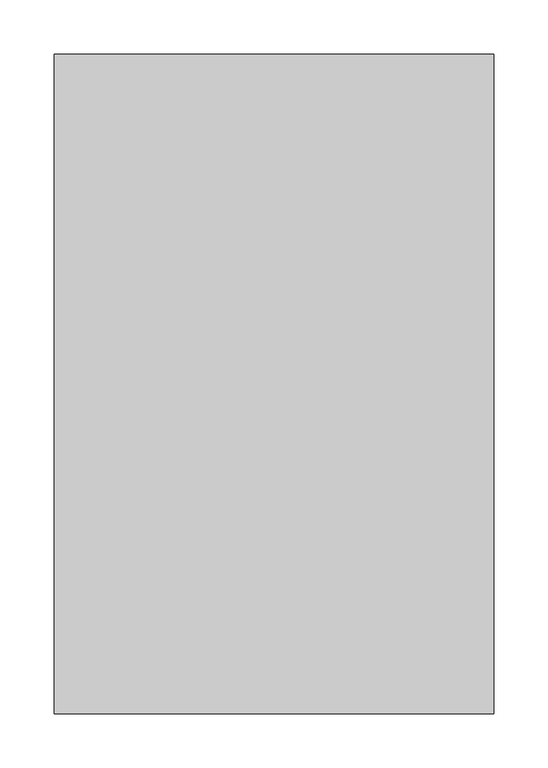
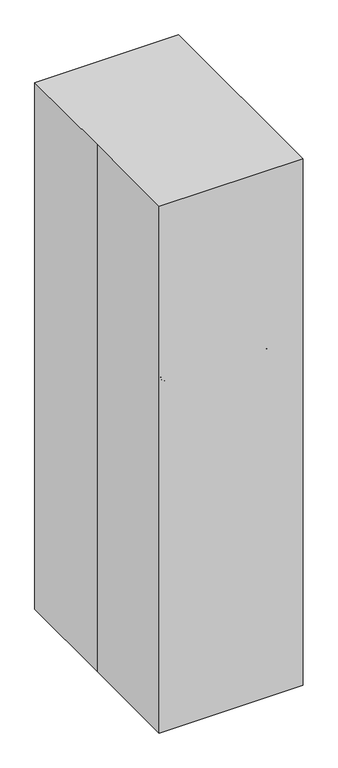
"""IFC4 building model written with IfcOpenShell, lengths in millimetres: proxy geometry, M8810 - Stand, Mayo : M8810 - Stand, Mayo."""

import ifcopenshell
import ifcopenshell.guid

model = None  # the IFC model being written
_history = None  # IfcOwnerHistory: only IFC2X3 demands one
_inside = {}  # id of a spatial element -> (the spatial element, [elements in it])
_under = {}  # id of a project, library or spatial element -> (it, [spatial elements below it])
_declared = {}  # id of a project -> (the project, [libraries it declares])
_typed = {}  # id of a type object -> (the type object, [elements of that type])
_made_of = {}  # id of a material, layer set ... -> (it, [elements and type objects made of it])


def new_model(schema):
    """Start an empty IFC model of exactly this schema.

    Asked for "IFC4X3", IfcOpenShell would pick the latest addendum, in which some entities
    have other attributes; the version numbers below select the first issue.
    IFC2X3 requires an IfcOwnerHistory on every rooted entity: one is made here for all.
    """
    global model, _history
    if schema == "IFC4X3":
        model = ifcopenshell.file(schema_version=(4, 3, 0, 0))
    else:
        model = ifcopenshell.file(schema=schema)
    _inside.clear()
    _under.clear()
    _declared.clear()
    _typed.clear()
    _made_of.clear()
    _history = None
    if model.schema == "IFC2X3":
        org = make("IfcOrganization", Name="unknown")
        user = make(
            "IfcPersonAndOrganization",
            ThePerson=make("IfcPerson", FamilyName="unknown"),
            TheOrganization=org,
        )
        app = make(
            "IfcApplication",
            ApplicationDeveloper=org,
            Version="unknown",
            ApplicationFullName="unknown",
            ApplicationIdentifier="unknown",
        )
        _history = make(
            "IfcOwnerHistory",
            OwningUser=user,
            OwningApplication=app,
            ChangeAction="ADDED",
            CreationDate=0,
        )
    return model


def make(cls, **values):
    """One entity of the class cls with the attributes given. An attribute that is None is left unset."""
    return model.create_entity(
        cls, **{name: value for name, value in values.items() if value is not None}
    )


def rooted(cls, **values):
    """An entity with a GlobalId (a new one), such as an element, a storey or a relation."""
    return make(cls, GlobalId=ifcopenshell.guid.new(), OwnerHistory=_history, **values)


def si_unit(unit_type, name, prefix=None):
    """IfcSIUnit, for example si_unit("LENGTHUNIT", "METRE", prefix="MILLI")."""
    return make("IfcSIUnit", UnitType=unit_type, Prefix=prefix, Name=name)


def assignment(units):
    """IfcUnitAssignment: the units of a project."""
    return None if units is None else make("IfcUnitAssignment", Units=units)


def point(xyz):
    """IfcCartesianPoint."""
    return None if xyz is None else make("IfcCartesianPoint", Coordinates=xyz)


def direction(xyz):
    """IfcDirection."""
    return None if xyz is None else make("IfcDirection", DirectionRatios=xyz)


def frame(location, z_axis=None, x_axis=None):
    """IfcAxis2Placement3D, a coordinate frame: its origin and axes. An axis left out is left unset."""
    return make(
        "IfcAxis2Placement3D",
        Location=point(location),
        Axis=direction(z_axis),
        RefDirection=direction(x_axis),
    )


def origin():
    """The frame at (0, 0, 0) with its axes left unset."""
    return frame((0.0, 0.0, 0.0))


def origin_with_axes():
    """The frame at (0, 0, 0) with the z axis (0, 0, 1) and the x axis (1, 0, 0) written out."""
    return frame((0.0, 0.0, 0.0), z_axis=(0.0, 0.0, 1.0), x_axis=(1.0, 0.0, 0.0))


def place(relative_to, where):
    """IfcLocalPlacement: puts the frame where relative to a parent placement (None: the world)."""
    return make(
        "IfcLocalPlacement", PlacementRelTo=relative_to, RelativePlacement=where
    )


def context(
    kind, dimensions, precision=None, world=None, true_north=None, identifier=None
):
    """IfcGeometricRepresentationContext, for example the 3D "Model" context."""
    return make(
        "IfcGeometricRepresentationContext",
        ContextIdentifier=identifier,
        ContextType=kind,
        CoordinateSpaceDimension=dimensions,
        Precision=precision,
        WorldCoordinateSystem=world,
        TrueNorth=true_north,
    )


def project(units=None, contexts=None):
    """IfcProject with its units and contexts."""
    return rooted(
        "IfcProject",
        Name="project",
        RepresentationContexts=contexts,
        UnitsInContext=assignment(units),
    )


def spatial(cls, under=None, at=None, **own):
    """A site, building, storey or space (cls), placed at a placement, below another one or the project."""
    s = rooted(cls, ObjectPlacement=at, **own)
    if under is not None:
        _under.setdefault(under.id(), (under, []))[1].append(s)
    return s


def polyline(points):
    """IfcPolyline through the points."""
    return make("IfcPolyline", Points=[point(p) for p in points])


def circle_curve(where, radius):
    """IfcCircle in the frame where."""
    return make("IfcCircle", Position=where, Radius=radius)


def ellipse_curve(where, semi_axis1, semi_axis2):
    """IfcEllipse in the frame where."""
    return make(
        "IfcEllipse", Position=where, SemiAxis1=semi_axis1, SemiAxis2=semi_axis2
    )


def trimmed(basis, trim1, trim2, sense, master):
    """IfcTrimmedCurve: the piece of a basis curve between two trims."""
    return make(
        "IfcTrimmedCurve",
        BasisCurve=basis,
        Trim1=trim1,
        Trim2=trim2,
        SenseAgreement=sense,
        MasterRepresentation=master,
    )


def outline(outer, holes=None, kind="AREA"):
    """IfcArbitraryClosedProfileDef: a profile drawn as a closed curve; with holes, ...WithVoids."""
    if holes is None:
        return make("IfcArbitraryClosedProfileDef", ProfileType=kind, OuterCurve=outer)
    return make(
        "IfcArbitraryProfileDefWithVoids",
        ProfileType=kind,
        OuterCurve=outer,
        InnerCurves=holes,
    )


def extrude(swept, where, along, depth):
    """IfcExtrudedAreaSolid: the profile swept, set in the frame where, extruded along a direction by depth."""
    return make(
        "IfcExtrudedAreaSolid",
        SweptArea=swept,
        Position=where,
        ExtrudedDirection=direction(along),
        Depth=depth,
    )


def shape(context_of_items, identifier, shape_type, items):
    """IfcShapeRepresentation: the items that make up one representation, for example the "Body"."""
    return make(
        "IfcShapeRepresentation",
        ContextOfItems=context_of_items,
        RepresentationIdentifier=identifier,
        RepresentationType=shape_type,
        Items=items,
    )


def source(mapping_origin, context_of_items, identifier, shape_type, items):
    """IfcRepresentationMap: a shape defined once, which mapped items show again and again."""
    return make(
        "IfcRepresentationMap",
        MappingOrigin=mapping_origin,
        MappedRepresentation=shape(context_of_items, identifier, shape_type, items),
    )


def transform(
    local_origin,
    x_axis=None,
    y_axis=None,
    z_axis=None,
    scale=None,
    scale2=None,
    scale3=None,
    uniform=True,
):
    """IfcCartesianTransformationOperator3D, or its non-uniform kind. x_axis, y_axis, z_axis: its Axis1, 2, 3."""
    if uniform:
        return make(
            "IfcCartesianTransformationOperator3D",
            Axis1=direction(x_axis),
            Axis2=direction(y_axis),
            LocalOrigin=point(local_origin),
            Scale=scale,
            Axis3=direction(z_axis),
        )
    return make(
        "IfcCartesianTransformationOperator3DnonUniform",
        Axis1=direction(x_axis),
        Axis2=direction(y_axis),
        LocalOrigin=point(local_origin),
        Scale=scale,
        Axis3=direction(z_axis),
        Scale2=scale2,
        Scale3=scale3,
    )


def mapped(mapping_source, mapping_target):
    """IfcMappedItem: shows the shape of a source again, moved by a transform."""
    return make(
        "IfcMappedItem", MappingSource=mapping_source, MappingTarget=mapping_target
    )


def made_of(thing, what):
    """Note that an element or type object is made of a material, layer set ...; save() writes the relation."""
    if what is not None:
        _made_of.setdefault(what.id(), (what, []))[1].append(thing)
    return thing


def element(
    cls,
    number,
    at=None,
    inside=None,
    cuts=None,
    type_object=None,
    material=None,
    context=None,
    identifier="Body",
    shape_type=None,
    held_by="IfcProductDefinitionShape",
    body=None,
    shapes=None,
    **own,
):
    """One element of the class cls, such as IfcWall. Its Tag is "e" and its number.

    at: its placement. inside: the storey or other place that contains it. cuts: it is an
    opening in that element (IfcRelVoidsElement). A single representation is given by context,
    identifier, shape_type and body (its items); several are given by shapes. held_by: the class
    of the entity that holds the representations. save() writes the other relations.
    """
    e = rooted(cls, Tag="e%d" % number, ObjectPlacement=at, **own)
    if body is not None:
        shapes = [shape(context, identifier, shape_type, body)]
    if shapes is not None:
        e.Representation = make(held_by, Representations=shapes)
    if inside is not None:
        _inside.setdefault(inside.id(), (inside, []))[1].append(e)
    if cuts is not None:
        rooted(
            "IfcRelVoidsElement", RelatingBuildingElement=cuts, RelatedOpeningElement=e
        )
    if type_object is not None:
        _typed.setdefault(type_object.id(), (type_object, []))[1].append(e)
    return made_of(e, material)


def aggregate(whole, parts):
    """IfcRelAggregates: a whole, such as a stair, and the parts it consists of."""
    return rooted("IfcRelAggregates", RelatingObject=whole, RelatedObjects=parts)


def save(model, path):
    """Write the relations noted so far, then the file.

    IfcRelAggregates (storeys below a building ...), IfcRelContainedInSpatialStructure (elements
    in a storey), IfcRelDefinesByType, IfcRelAssociatesMaterial and IfcRelDeclares: one each for
    every whole, place, type object, material and project.
    """
    for whole, parts in _under.values():
        aggregate(whole, parts)
    for where, things in _inside.values():
        rooted(
            "IfcRelContainedInSpatialStructure",
            RelatedElements=things,
            RelatingStructure=where,
        )
    for kind, things in _typed.values():
        rooted("IfcRelDefinesByType", RelatedObjects=things, RelatingType=kind)
    for what, things in _made_of.values():
        rooted("IfcRelAssociatesMaterial", RelatedObjects=things, RelatingMaterial=what)
    for by, libraries in _declared.values():
        rooted("IfcRelDeclares", RelatingContext=by, RelatedDefinitions=libraries)
    model.write(path)


def plane_surface(at):
    """IfcPlane: the flat surface through the origin of the frame at, square to its z axis."""
    return make("IfcPlane", Position=at)


def cylinder_surface(at, radius):
    """IfcCylindricalSurface: all points at the distance radius from the z axis of the frame at."""
    return make("IfcCylindricalSurface", Position=at, Radius=radius)


def revolved_surface(curve, axis_point, axis_direction):
    """IfcSurfaceOfRevolution: the curve turned about the line through axis_point along axis_direction."""
    return make(
        "IfcSurfaceOfRevolution",
        SweptCurve=make("IfcArbitraryOpenProfileDef", ProfileType="CURVE", Curve=curve),
        AxisPosition=make("IfcAxis1Placement", Location=point(axis_point), Axis=direction(axis_direction)),
    )


def advanced_brep(points, edges, surfaces, faces):
    """IfcAdvancedBrep: a solid bounded by faces that lie on surfaces and meet in shared edges.

    An edge is (start, end): straight between two places in points (the first is 0);
    or (start, end, curve); or (start, end, curve, False) where it runs against its curve.
    A face is (place in surfaces, loops), or (place, loops, False) where it looks against
    its surface's normal. A loop lists edges by number (the first is 1), with a minus sign
    where the edge is run from its end to its start. The first loop is the outer one.
    """
    corners = [point(p) for p in points]
    vertices = [make("IfcVertexPoint", VertexGeometry=c) for c in corners]
    made = []
    for start, end, *more in edges:
        made.append(
            make(
                "IfcEdgeCurve",
                EdgeStart=vertices[start],
                EdgeEnd=vertices[end],
                EdgeGeometry=more[0] if more else make("IfcPolyline", Points=[corners[start], corners[end]]),
                SameSense=more[1] if len(more) > 1 else True,
            )
        )
    hull = []
    for where, loops, *sense in faces:
        bounds = []
        for j, loop in enumerate(loops):
            ring = [make("IfcOrientedEdge", EdgeElement=made[abs(k) - 1], Orientation=k > 0) for k in loop]
            bounds.append(
                make(
                    "IfcFaceOuterBound" if j == 0 else "IfcFaceBound",
                    Bound=make("IfcEdgeLoop", EdgeList=ring),
                    Orientation=True,
                )
            )
        hull.append(make("IfcAdvancedFace", Bounds=bounds, FaceSurface=surfaces[where], SameSense=sense[0] if sense else True))
    return make("IfcAdvancedBrep", Outer=make("IfcClosedShell", CfsFaces=hull))


def specialty_equipment_9fd3930d(model_context):
    return source(origin(), model_context, "Body", "SolidModel", [
        advanced_brep(
        [(-123.5140783, 201.8552552, 999.8159151), (-136.2140783, 189.1552552, 999.8159151), (-136.2140783, 189.1552552, 996.6409151), (-123.5140783, 201.8552552, 996.6409151), (-123.5140783, 224.0802552, 1002.9909151), (-158.4390783, 189.1552552, 1002.9909151), (-155.2640783, 189.1552552, 999.8159151), (-123.5140783, 220.9052552, 999.8159151), (-123.5140783, 224.0802552, 1015.2574617), (-158.4390783, 189.1552552, 1015.2574617), (-123.5140783, 226.4102935, 1017.5875), (-160.7691166, 189.1552552, 1017.5875), (-123.5140783, 233.6052552, 1015.5808485), (-167.9640783, 189.1552552, 1015.5808485), (-165.9574268, 189.1552552, 1017.5875), (-123.5140783, 231.5986038, 1017.5875), (-123.5140783, 233.6052552, 1011.9917262), (-167.9640783, 189.1552552, 1011.9917262), (-123.5140783, 232.8510291, 1011.2375), (-167.2098521, 189.1552552, 1011.2375), (-123.5140783, 232.0177552, 1016.0), (-166.3765783, 189.1552552, 1016.0), (-166.3765783, 189.1552552, 1011.2375), (-123.5140783, 232.0177552, 1011.2375), (-123.5140783, 227.2552552, 1002.9909151), (-161.6140783, 189.1552552, 1002.9909151), (-161.6140783, 189.1552552, 1016.0), (-123.5140783, 227.2552552, 1016.0), (-123.5140783, 220.9052552, 996.6409151), (-155.2640783, 189.1552552, 996.6409151), (124.1359217, 201.8552552, 996.6409151), (124.1359217, 201.8552552, 999.8159151), (124.1359217, 220.9052552, 999.8159151), (124.1359217, 224.0802552, 1002.9909151), (124.1359217, 224.0802552, 1015.2574617), (124.1359217, 226.4102935, 1017.5875), (124.1359217, 231.5986038, 1017.5875), (124.1359217, 233.6052552, 1015.5808485), (124.1359217, 233.6052552, 1011.9917262), (124.1359217, 232.8510291, 1011.2375), (124.1359217, 232.0177552, 1011.2375), (124.1359217, 232.0177552, 1016.0), (124.1359217, 227.2552552, 1016.0), (124.1359217, 227.2552552, 1002.9909151), (124.1359217, 220.9052552, 996.6409151), (136.8359217, 189.1552552, 999.8159151), (136.8359217, 189.1552552, 996.6409151), (159.0609217, 189.1552552, 1002.9909151), (155.8859217, 189.1552552, 999.8159151), (159.0609217, 189.1552552, 1015.2574617), (161.39096, 189.1552552, 1017.5875), (168.5859217, 189.1552552, 1015.5808485), (166.5792702, 189.1552552, 1017.5875), (168.5859217, 189.1552552, 1011.9917262), (167.8316955, 189.1552552, 1011.2375), (166.9984217, 189.1552552, 1016.0), (166.9984217, 189.1552552, 1011.2375), (162.2359217, 189.1552552, 1002.9909151), (162.2359217, 189.1552552, 1016.0), (155.8859217, 189.1552552, 996.6409151), (136.8359217, -223.5947448, 996.6409151), (136.8359217, -223.5947448, 999.8159151), (155.8859217, -223.5947448, 999.8159151), (159.0609217, -223.5947448, 1002.9909151), (159.0609217, -223.5947448, 1015.2574617), (161.39096, -223.5947448, 1017.5875), (166.5792702, -223.5947448, 1017.5875), (168.5859217, -223.5947448, 1015.5808485), (168.5859217, -223.5947448, 1011.9917262), (167.8316955, -223.5947448, 1011.2375), (166.9984217, -223.5947448, 1011.2375), (166.9984217, -223.5947448, 1016.0), (162.2359217, -223.5947448, 1016.0), (162.2359217, -223.5947448, 1002.9909151), (155.8859217, -223.5947448, 996.6409151), (124.1359217, -236.2947448, 999.8159151), (124.1359217, -236.2947448, 996.6409151), (124.1359217, -258.5197448, 1002.9909151), (124.1359217, -255.3447448, 999.8159151), (124.1359217, -258.5197448, 1015.2574617), (124.1359217, -260.849783, 1017.5875), (124.1359217, -268.0447448, 1015.5808485), (124.1359217, -266.0380933, 1017.5875), (124.1359217, -268.0447448, 1011.9917262), (124.1359217, -267.2905186, 1011.2375), (124.1359217, -266.4572448, 1016.0), (124.1359217, -266.4572448, 1011.2375), (124.1359217, -261.6947448, 1002.9909151), (124.1359217, -261.6947448, 1016.0), (124.1359217, -255.3447448, 996.6409151), (-123.5140783, -236.2947448, 996.6409151), (-123.5140783, -236.2947448, 999.8159151), (-123.5140783, -255.3447448, 999.8159151), (-123.5140783, -258.5197448, 1002.9909151), (-123.5140783, -258.5197448, 1015.2574617), (-123.5140783, -260.849783, 1017.5875), (-123.5140783, -266.0380933, 1017.5875), (-123.5140783, -268.0447448, 1015.5808485), (-123.5140783, -268.0447448, 1011.9917262), (-123.5140783, -267.2905186, 1011.2375), (-123.5140783, -266.4572448, 1011.2375), (-123.5140783, -266.4572448, 1016.0), (-123.5140783, -261.6947448, 1016.0), (-123.5140783, -261.6947448, 1002.9909151), (-123.5140783, -255.3447448, 996.6409151), (-136.2140783, -223.5947448, 999.8159151), (-136.2140783, -223.5947448, 996.6409151), (-155.2640783, -223.5947448, 999.8159151), (-158.4390783, -223.5947448, 1002.9909151), (-158.4390783, -223.5947448, 1015.2574617), (-160.7691166, -223.5947448, 1017.5875), (-165.9574268, -223.5947448, 1017.5875), (-167.9640783, -223.5947448, 1015.5808485), (-167.9640783, -223.5947448, 1011.9917262), (-167.2098521, -223.5947448, 1011.2375), (-166.3765783, -223.5947448, 1011.2375), (-166.3765783, -223.5947448, 1016.0), (-161.6140783, -223.5947448, 1016.0), (-161.6140783, -223.5947448, 1002.9909151), (-155.2640783, -223.5947448, 996.6409151)],
        [
            (0, 1, circle_curve(frame((-123.5140783, 189.1552552, 999.8159151), z_axis=(0.0, 0.0, 1.0), x_axis=(-1.0, 0.0, 0.0)), 12.7)),
            (1, 2),
            (2, 3, circle_curve(frame((-123.5140783, 189.1552552, 996.6409151), z_axis=(0.0, 0.0, -1.0), x_axis=(-1.0, 0.0, 0.0)), 12.7)),
            (3, 0),
            (4, 5, circle_curve(frame((-123.5140783, 189.1552552, 1002.9909151), z_axis=(0.0, 0.0, 1.0), x_axis=(-1.0, 0.0, 0.0)), 34.925)),
            (5, 6, circle_curve(frame((-155.2640783, 189.1552552, 1002.9909151), z_axis=(0.0, -1.0, 0.0), x_axis=(-1.0, 0.0, 0.0)), 3.175)),
            (6, 7, circle_curve(frame((-123.5140783, 189.1552552, 999.8159151), z_axis=(0.0, 0.0, -1.0), x_axis=(-1.0, 0.0, 0.0)), 31.75)),
            (7, 4, circle_curve(frame((-123.5140783, 220.9052552, 1002.9909151), z_axis=(1.0, 0.0, 0.0), x_axis=(0.0, 1.0, 0.0)), 3.175)),
            (8, 9, circle_curve(frame((-123.5140783, 189.1552552, 1015.2574617), z_axis=(0.0, 0.0, 1.0), x_axis=(-1.0, 0.0, 0.0)), 34.925)),
            (9, 5),
            (4, 8),
            (10, 11, circle_curve(frame((-123.5140783, 189.1552552, 1017.5875), z_axis=(0.0, 0.0, 1.0), x_axis=(-1.0, 0.0, 0.0)), 37.2550383)),
            (11, 9, circle_curve(frame((-160.7691166, 189.1552552, 1015.2574617), z_axis=(0.0, 1.0, 0.0), x_axis=(-1.0, 0.0, 0.0)), 2.3300383)),
            (8, 10, circle_curve(frame((-123.5140783, 226.4102935, 1015.2574617), z_axis=(-1.0, 0.0, 0.0), x_axis=(0.0, 1.0, 0.0)), 2.3300383)),
            (12, 13, circle_curve(frame((-123.5140783, 189.1552552, 1015.5808485), z_axis=(0.0, 0.0, 1.0), x_axis=(-1.0, 0.0, 0.0)), 44.45)),
            (13, 14, circle_curve(frame((-165.9574268, 189.1552552, 1015.5808485), z_axis=(0.0, 1.0, 0.0), x_axis=(-1.0, 0.0, 0.0)), 2.0066515)),
            (14, 15, circle_curve(frame((-123.5140783, 189.1552552, 1017.5875), z_axis=(0.0, 0.0, -1.0), x_axis=(-1.0, 0.0, 0.0)), 42.4433485)),
            (15, 12, circle_curve(frame((-123.5140783, 231.5986038, 1015.5808485), z_axis=(-1.0, 0.0, 0.0), x_axis=(0.0, 1.0, 0.0)), 2.0066515)),
            (16, 17, circle_curve(frame((-123.5140783, 189.1552552, 1011.9917262), z_axis=(0.0, 0.0, 1.0), x_axis=(-1.0, 0.0, 0.0)), 44.45)),
            (17, 13),
            (12, 16),
            (18, 19, circle_curve(frame((-123.5140783, 189.1552552, 1011.2375), z_axis=(0.0, 0.0, 1.0), x_axis=(-1.0, 0.0, 0.0)), 43.6957738)),
            (19, 17, circle_curve(frame((-167.2098521, 189.1552552, 1011.9917262), z_axis=(0.0, 1.0, 0.0), x_axis=(-1.0, 0.0, 0.0)), 0.7542262)),
            (16, 18, circle_curve(frame((-123.5140783, 232.8510291, 1011.9917262), z_axis=(-1.0, 0.0, 0.0), x_axis=(0.0, 1.0, 0.0)), 0.7542262)),
            (20, 21, circle_curve(frame((-123.5140783, 189.1552552, 1016.0), z_axis=(0.0, 0.0, 1.0), x_axis=(-1.0, 0.0, 0.0)), 42.8625)),
            (21, 22),
            (22, 23, circle_curve(frame((-123.5140783, 189.1552552, 1011.2375), z_axis=(0.0, 0.0, -1.0), x_axis=(-1.0, 0.0, 0.0)), 42.8625)),
            (23, 20),
            (24, 25, circle_curve(frame((-123.5140783, 189.1552552, 1002.9909151), z_axis=(0.0, 0.0, 1.0), x_axis=(-1.0, 0.0, 0.0)), 38.1)),
            (25, 26),
            (26, 27, circle_curve(frame((-123.5140783, 189.1552552, 1016.0), z_axis=(0.0, 0.0, -1.0), x_axis=(-1.0, 0.0, 0.0)), 38.1)),
            (27, 24),
            (28, 29, circle_curve(frame((-123.5140783, 189.1552552, 996.6409151), z_axis=(0.0, 0.0, 1.0), x_axis=(-1.0, 0.0, 0.0)), 31.75)),
            (29, 25, circle_curve(frame((-155.2640783, 189.1552552, 1002.9909151), z_axis=(0.0, 1.0, 0.0), x_axis=(-1.0, 0.0, 0.0)), 6.35)),
            (24, 28, circle_curve(frame((-123.5140783, 220.9052552, 1002.9909151), z_axis=(-1.0, 0.0, 0.0), x_axis=(0.0, 1.0, 0.0)), 6.35)),
            (3, 30),
            (30, 31),
            (31, 0),
            (7, 32),
            (32, 33, circle_curve(frame((124.1359217, 220.9052552, 1002.9909151), z_axis=(1.0, 0.0, 0.0), x_axis=(0.0, 1.0, 0.0)), 3.175)),
            (33, 4),
            (33, 34),
            (34, 8),
            (34, 35, circle_curve(frame((124.1359217, 226.4102935, 1015.2574617), z_axis=(-1.0, 0.0, 0.0), x_axis=(0.0, 1.0, 0.0)), 2.3300383)),
            (35, 10),
            (15, 36),
            (36, 37, circle_curve(frame((124.1359217, 231.5986038, 1015.5808485), z_axis=(-1.0, 0.0, 0.0), x_axis=(0.0, 1.0, 0.0)), 2.0066515)),
            (37, 12),
            (37, 38),
            (38, 16),
            (38, 39, circle_curve(frame((124.1359217, 232.8510291, 1011.9917262), z_axis=(-1.0, 0.0, 0.0), x_axis=(0.0, 1.0, 0.0)), 0.7542262)),
            (39, 18),
            (23, 40),
            (40, 41),
            (41, 20),
            (27, 42),
            (42, 43),
            (43, 24),
            (43, 44, circle_curve(frame((124.1359217, 220.9052552, 1002.9909151), z_axis=(-1.0, 0.0, 0.0), x_axis=(0.0, 1.0, 0.0)), 6.35)),
            (44, 28),
            (45, 31, circle_curve(frame((124.1359217, 189.1552552, 999.8159151), z_axis=(0.0, 0.0, 1.0), x_axis=(0.0, 1.0, 0.0)), 12.7)),
            (30, 46, circle_curve(frame((124.1359217, 189.1552552, 996.6409151), z_axis=(0.0, 0.0, -1.0), x_axis=(0.0, 1.0, 0.0)), 12.7)),
            (46, 45),
            (47, 33, circle_curve(frame((124.1359217, 189.1552552, 1002.9909151), z_axis=(0.0, 0.0, 1.0), x_axis=(0.0, 1.0, 0.0)), 34.925)),
            (32, 48, circle_curve(frame((124.1359217, 189.1552552, 999.8159151), z_axis=(0.0, 0.0, -1.0), x_axis=(0.0, 1.0, 0.0)), 31.75)),
            (48, 47, circle_curve(frame((155.8859217, 189.1552552, 1002.9909151), z_axis=(0.0, -1.0, 0.0), x_axis=(1.0, 0.0, 0.0)), 3.175)),
            (49, 34, circle_curve(frame((124.1359217, 189.1552552, 1015.2574617), z_axis=(0.0, 0.0, 1.0), x_axis=(0.0, 1.0, 0.0)), 34.925)),
            (47, 49),
            (50, 35, circle_curve(frame((124.1359217, 189.1552552, 1017.5875), z_axis=(0.0, 0.0, 1.0), x_axis=(0.0, 1.0, 0.0)), 37.2550383)),
            (49, 50, circle_curve(frame((161.39096, 189.1552552, 1015.2574617), z_axis=(0.0, 1.0, 0.0), x_axis=(1.0, 0.0, 0.0)), 2.3300383)),
            (51, 37, circle_curve(frame((124.1359217, 189.1552552, 1015.5808485), z_axis=(0.0, 0.0, 1.0), x_axis=(0.0, 1.0, 0.0)), 44.45)),
            (36, 52, circle_curve(frame((124.1359217, 189.1552552, 1017.5875), z_axis=(0.0, 0.0, -1.0), x_axis=(0.0, 1.0, 0.0)), 42.4433485)),
            (52, 51, circle_curve(frame((166.5792702, 189.1552552, 1015.5808485), z_axis=(0.0, 1.0, 0.0), x_axis=(1.0, 0.0, 0.0)), 2.0066515)),
            (53, 38, circle_curve(frame((124.1359217, 189.1552552, 1011.9917262), z_axis=(0.0, 0.0, 1.0), x_axis=(0.0, 1.0, 0.0)), 44.45)),
            (51, 53),
            (54, 39, circle_curve(frame((124.1359217, 189.1552552, 1011.2375), z_axis=(0.0, 0.0, 1.0), x_axis=(0.0, 1.0, 0.0)), 43.6957738)),
            (53, 54, circle_curve(frame((167.8316955, 189.1552552, 1011.9917262), z_axis=(0.0, 1.0, 0.0), x_axis=(1.0, 0.0, 0.0)), 0.7542262)),
            (55, 41, circle_curve(frame((124.1359217, 189.1552552, 1016.0), z_axis=(0.0, 0.0, 1.0), x_axis=(0.0, 1.0, 0.0)), 42.8625)),
            (40, 56, circle_curve(frame((124.1359217, 189.1552552, 1011.2375), z_axis=(0.0, 0.0, -1.0), x_axis=(0.0, 1.0, 0.0)), 42.8625)),
            (56, 55),
            (57, 43, circle_curve(frame((124.1359217, 189.1552552, 1002.9909151), z_axis=(0.0, 0.0, 1.0), x_axis=(0.0, 1.0, 0.0)), 38.1)),
            (42, 58, circle_curve(frame((124.1359217, 189.1552552, 1016.0), z_axis=(0.0, 0.0, -1.0), x_axis=(0.0, 1.0, 0.0)), 38.1)),
            (58, 57),
            (59, 44, circle_curve(frame((124.1359217, 189.1552552, 996.6409151), z_axis=(0.0, 0.0, 1.0), x_axis=(0.0, 1.0, 0.0)), 31.75)),
            (57, 59, circle_curve(frame((155.8859217, 189.1552552, 1002.9909151), z_axis=(0.0, 1.0, 0.0), x_axis=(1.0, 0.0, 0.0)), 6.35)),
            (46, 60),
            (60, 61),
            (61, 45),
            (48, 62),
            (62, 63, circle_curve(frame((155.8859217, -223.5947448, 1002.9909151), z_axis=(0.0, -1.0, 0.0), x_axis=(1.0, 0.0, 0.0)), 3.175)),
            (63, 47),
            (63, 64),
            (64, 49),
            (64, 65, circle_curve(frame((161.39096, -223.5947448, 1015.2574617), z_axis=(0.0, 1.0, 0.0), x_axis=(1.0, 0.0, 0.0)), 2.3300383)),
            (65, 50),
            (52, 66),
            (66, 67, circle_curve(frame((166.5792702, -223.5947448, 1015.5808485), z_axis=(0.0, 1.0, 0.0), x_axis=(1.0, 0.0, 0.0)), 2.0066515)),
            (67, 51),
            (67, 68),
            (68, 53),
            (68, 69, circle_curve(frame((167.8316955, -223.5947448, 1011.9917262), z_axis=(0.0, 1.0, 0.0), x_axis=(1.0, 0.0, 0.0)), 0.7542262)),
            (69, 54),
            (56, 70),
            (70, 71),
            (71, 55),
            (58, 72),
            (72, 73),
            (73, 57),
            (73, 74, circle_curve(frame((155.8859217, -223.5947448, 1002.9909151), z_axis=(0.0, 1.0, 0.0), x_axis=(1.0, 0.0, 0.0)), 6.35)),
            (74, 59),
            (75, 61, circle_curve(frame((124.1359217, -223.5947448, 999.8159151), z_axis=(0.0, 0.0, 1.0), x_axis=(1.0, 0.0, 0.0)), 12.7)),
            (60, 76, circle_curve(frame((124.1359217, -223.5947448, 996.6409151), z_axis=(0.0, 0.0, -1.0), x_axis=(1.0, 0.0, 0.0)), 12.7)),
            (76, 75),
            (77, 63, circle_curve(frame((124.1359217, -223.5947448, 1002.9909151), z_axis=(0.0, 0.0, 1.0), x_axis=(1.0, 0.0, 0.0)), 34.925)),
            (62, 78, circle_curve(frame((124.1359217, -223.5947448, 999.8159151), z_axis=(0.0, 0.0, -1.0), x_axis=(1.0, 0.0, 0.0)), 31.75)),
            (78, 77, circle_curve(frame((124.1359217, -255.3447448, 1002.9909151), z_axis=(-1.0, 0.0, 0.0), x_axis=(0.0, -1.0, 0.0)), 3.175)),
            (79, 64, circle_curve(frame((124.1359217, -223.5947448, 1015.2574617), z_axis=(0.0, 0.0, 1.0), x_axis=(1.0, 0.0, 0.0)), 34.925)),
            (77, 79),
            (80, 65, circle_curve(frame((124.1359217, -223.5947448, 1017.5875), z_axis=(0.0, 0.0, 1.0), x_axis=(1.0, 0.0, 0.0)), 37.2550383)),
            (79, 80, circle_curve(frame((124.1359217, -260.849783, 1015.2574617), z_axis=(1.0, 0.0, 0.0), x_axis=(0.0, -1.0, 0.0)), 2.3300383)),
            (81, 67, circle_curve(frame((124.1359217, -223.5947448, 1015.5808485), z_axis=(0.0, 0.0, 1.0), x_axis=(1.0, 0.0, 0.0)), 44.45)),
            (66, 82, circle_curve(frame((124.1359217, -223.5947448, 1017.5875), z_axis=(0.0, 0.0, -1.0), x_axis=(1.0, 0.0, 0.0)), 42.4433485)),
            (82, 81, circle_curve(frame((124.1359217, -266.0380933, 1015.5808485), z_axis=(1.0, 0.0, 0.0), x_axis=(0.0, -1.0, 0.0)), 2.0066515)),
            (83, 68, circle_curve(frame((124.1359217, -223.5947448, 1011.9917262), z_axis=(0.0, 0.0, 1.0), x_axis=(1.0, 0.0, 0.0)), 44.45)),
            (81, 83),
            (84, 69, circle_curve(frame((124.1359217, -223.5947448, 1011.2375), z_axis=(0.0, 0.0, 1.0), x_axis=(1.0, 0.0, 0.0)), 43.6957738)),
            (83, 84, circle_curve(frame((124.1359217, -267.2905186, 1011.9917262), z_axis=(1.0, 0.0, 0.0), x_axis=(0.0, -1.0, 0.0)), 0.7542262)),
            (85, 71, circle_curve(frame((124.1359217, -223.5947448, 1016.0), z_axis=(0.0, 0.0, 1.0), x_axis=(1.0, 0.0, 0.0)), 42.8625)),
            (70, 86, circle_curve(frame((124.1359217, -223.5947448, 1011.2375), z_axis=(0.0, 0.0, -1.0), x_axis=(1.0, 0.0, 0.0)), 42.8625)),
            (86, 85),
            (87, 73, circle_curve(frame((124.1359217, -223.5947448, 1002.9909151), z_axis=(0.0, 0.0, 1.0), x_axis=(1.0, 0.0, 0.0)), 38.1)),
            (72, 88, circle_curve(frame((124.1359217, -223.5947448, 1016.0), z_axis=(0.0, 0.0, -1.0), x_axis=(1.0, 0.0, 0.0)), 38.1)),
            (88, 87),
            (89, 74, circle_curve(frame((124.1359217, -223.5947448, 996.6409151), z_axis=(0.0, 0.0, 1.0), x_axis=(1.0, 0.0, 0.0)), 31.75)),
            (87, 89, circle_curve(frame((124.1359217, -255.3447448, 1002.9909151), z_axis=(1.0, 0.0, 0.0), x_axis=(0.0, -1.0, 0.0)), 6.35)),
            (76, 90),
            (90, 91),
            (91, 75),
            (78, 92),
            (92, 93, circle_curve(frame((-123.5140783, -255.3447448, 1002.9909151), z_axis=(-1.0, 0.0, 0.0), x_axis=(0.0, -1.0, 0.0)), 3.175)),
            (93, 77),
            (93, 94),
            (94, 79),
            (94, 95, circle_curve(frame((-123.5140783, -260.849783, 1015.2574617), z_axis=(1.0, 0.0, 0.0), x_axis=(0.0, -1.0, 0.0)), 2.3300383)),
            (95, 80),
            (82, 96),
            (96, 97, circle_curve(frame((-123.5140783, -266.0380933, 1015.5808485), z_axis=(1.0, 0.0, 0.0), x_axis=(0.0, -1.0, 0.0)), 2.0066515)),
            (97, 81),
            (97, 98),
            (98, 83),
            (98, 99, circle_curve(frame((-123.5140783, -267.2905186, 1011.9917262), z_axis=(1.0, 0.0, 0.0), x_axis=(0.0, -1.0, 0.0)), 0.7542262)),
            (99, 84),
            (86, 100),
            (100, 101),
            (101, 85),
            (88, 102),
            (102, 103),
            (103, 87),
            (103, 104, circle_curve(frame((-123.5140783, -255.3447448, 1002.9909151), z_axis=(1.0, 0.0, 0.0), x_axis=(0.0, -1.0, 0.0)), 6.35)),
            (104, 89),
            (105, 91, circle_curve(frame((-123.5140783, -223.5947448, 999.8159151), z_axis=(0.0, 0.0, 1.0), x_axis=(0.0, -1.0, 0.0)), 12.7)),
            (90, 106, circle_curve(frame((-123.5140783, -223.5947448, 996.6409151), z_axis=(0.0, 0.0, -1.0), x_axis=(0.0, -1.0, 0.0)), 12.7)),
            (106, 105),
            (107, 92, circle_curve(frame((-123.5140783, -223.5947448, 999.8159151), z_axis=(0.0, 0.0, 1.0), x_axis=(0.0, -1.0, 0.0)), 31.75)),
            (6, 107),
            (105, 1),
            (108, 93, circle_curve(frame((-123.5140783, -223.5947448, 1002.9909151), z_axis=(0.0, 0.0, 1.0), x_axis=(0.0, -1.0, 0.0)), 34.925)),
            (107, 108, circle_curve(frame((-155.2640783, -223.5947448, 1002.9909151), z_axis=(0.0, 1.0, 0.0), x_axis=(-1.0, 0.0, 0.0)), 3.175)),
            (109, 94, circle_curve(frame((-123.5140783, -223.5947448, 1015.2574617), z_axis=(0.0, 0.0, 1.0), x_axis=(0.0, -1.0, 0.0)), 34.925)),
            (108, 109),
            (110, 95, circle_curve(frame((-123.5140783, -223.5947448, 1017.5875), z_axis=(0.0, 0.0, 1.0), x_axis=(0.0, -1.0, 0.0)), 37.2550383)),
            (109, 110, circle_curve(frame((-160.7691166, -223.5947448, 1015.2574617), z_axis=(0.0, -1.0, 0.0), x_axis=(-1.0, 0.0, 0.0)), 2.3300383)),
            (111, 96, circle_curve(frame((-123.5140783, -223.5947448, 1017.5875), z_axis=(0.0, 0.0, 1.0), x_axis=(0.0, -1.0, 0.0)), 42.4433485)),
            (14, 111),
            (110, 11),
            (112, 97, circle_curve(frame((-123.5140783, -223.5947448, 1015.5808485), z_axis=(0.0, 0.0, 1.0), x_axis=(0.0, -1.0, 0.0)), 44.45)),
            (111, 112, circle_curve(frame((-165.9574268, -223.5947448, 1015.5808485), z_axis=(0.0, -1.0, 0.0), x_axis=(-1.0, 0.0, 0.0)), 2.0066515)),
            (113, 98, circle_curve(frame((-123.5140783, -223.5947448, 1011.9917262), z_axis=(0.0, 0.0, 1.0), x_axis=(0.0, -1.0, 0.0)), 44.45)),
            (112, 113),
            (114, 99, circle_curve(frame((-123.5140783, -223.5947448, 1011.2375), z_axis=(0.0, 0.0, 1.0), x_axis=(0.0, -1.0, 0.0)), 43.6957738)),
            (113, 114, circle_curve(frame((-167.2098521, -223.5947448, 1011.9917262), z_axis=(0.0, -1.0, 0.0), x_axis=(-1.0, 0.0, 0.0)), 0.7542262)),
            (114, 19),
            (115, 100, circle_curve(frame((-123.5140783, -223.5947448, 1011.2375), z_axis=(0.0, 0.0, 1.0), x_axis=(0.0, -1.0, 0.0)), 42.8625)),
            (22, 115),
            (116, 101, circle_curve(frame((-123.5140783, -223.5947448, 1016.0), z_axis=(0.0, 0.0, 1.0), x_axis=(0.0, -1.0, 0.0)), 42.8625)),
            (115, 116),
            (116, 21),
            (117, 102, circle_curve(frame((-123.5140783, -223.5947448, 1016.0), z_axis=(0.0, 0.0, 1.0), x_axis=(0.0, -1.0, 0.0)), 38.1)),
            (26, 117),
            (118, 103, circle_curve(frame((-123.5140783, -223.5947448, 1002.9909151), z_axis=(0.0, 0.0, 1.0), x_axis=(0.0, -1.0, 0.0)), 38.1)),
            (117, 118),
            (119, 104, circle_curve(frame((-123.5140783, -223.5947448, 996.6409151), z_axis=(0.0, 0.0, 1.0), x_axis=(0.0, -1.0, 0.0)), 31.75)),
            (118, 119, circle_curve(frame((-155.2640783, -223.5947448, 1002.9909151), z_axis=(0.0, -1.0, 0.0), x_axis=(-1.0, 0.0, 0.0)), 6.35)),
            (119, 29),
            (2, 106),
            (5, 108),
            (9, 109),
            (13, 112),
            (17, 113),
            (25, 118),
        ],
        [
            revolved_surface(polyline([(-136.21407829999998, 189.1552552, 996.6409151), (-136.21407829999998, 189.1552552, 999.8159151)]), (-123.5140783, 189.1552552, 977.5909151), (0.0, 0.0, -1.0)),
            revolved_surface(trimmed(ellipse_curve(frame((-155.2640783, 189.1552552, 1002.9909151), z_axis=(0.0, 1.0, 0.0), x_axis=(-1.0, 0.0, 0.0)), 3.175, 3.175), [point((-155.2640783, 189.1552552, 999.8159151))], [point((-158.4390783, 189.1552552, 1002.9909151))], True, "CARTESIAN"), (-123.5140783, 189.1552552, 977.5909151), (0.0, 0.0, -1.0)),
            revolved_surface(polyline([(-158.4390783, 189.1552552, 1002.9909151), (-158.4390783, 189.1552552, 1015.2574617)]), (-123.5140783, 189.1552552, 977.5909151), (0.0, 0.0, -1.0)),
            revolved_surface(trimmed(ellipse_curve(frame((-160.7691166, 189.1552552, 1015.2574617), z_axis=(0.0, -1.0, 0.0), x_axis=(-1.0, 0.0, 0.0)), 2.3300383, 2.3300383), [point((-158.4390783, 189.1552552, 1015.2574617))], [point((-160.7691166, 189.1552552, 1017.5875))], True, "CARTESIAN"), (-123.5140783, 189.1552552, 977.5909151), (0.0, 0.0, -1.0)),
            revolved_surface(trimmed(ellipse_curve(frame((-165.9574268, 189.1552552, 1015.5808485), z_axis=(0.0, -1.0, 0.0), x_axis=(-1.0, 0.0, 0.0)), 2.0066515, 2.0066515), [point((-165.9574268, 189.1552552, 1017.5875))], [point((-167.9640783, 189.1552552, 1015.5808485))], True, "CARTESIAN"), (-123.5140783, 189.1552552, 977.5909151), (0.0, 0.0, -1.0)),
            cylinder_surface(frame((-123.5140783, 189.1552552, 977.5909151), z_axis=(0.0, 0.0, -1.0), x_axis=(-1.0, 0.0, 0.0)), 44.45),
            revolved_surface(trimmed(ellipse_curve(frame((-167.2098521, 189.1552552, 1011.9917262), z_axis=(0.0, -1.0, 0.0), x_axis=(-1.0, 0.0, 0.0)), 0.7542262, 0.7542262), [point((-167.9640783, 189.1552552, 1011.9917262))], [point((-167.2098521, 189.1552552, 1011.2375))], True, "CARTESIAN"), (-123.5140783, 189.1552552, 977.5909151), (0.0, 0.0, -1.0)),
            revolved_surface(polyline([(-166.3765783, 189.1552552, 1011.2375), (-166.3765783, 189.1552552, 1016.0)]), (-123.5140783, 189.1552552, 977.5909151), (0.0, 0.0, -1.0)),
            cylinder_surface(frame((-123.5140783, 189.1552552, 977.5909151), z_axis=(0.0, 0.0, -1.0), x_axis=(-1.0, 0.0, 0.0)), 38.1),
            revolved_surface(trimmed(ellipse_curve(frame((-155.2640783, 189.1552552, 1002.9909151), z_axis=(0.0, -1.0, 0.0), x_axis=(-1.0, 0.0, 0.0)), 6.35, 6.35), [point((-161.6140783, 189.1552552, 1002.9909151))], [point((-155.2640783, 189.1552552, 996.6409151))], True, "CARTESIAN"), (-123.5140783, 189.1552552, 977.5909151), (0.0, 0.0, -1.0)),
            plane_surface(frame((-123.5140783, 201.8552552, 996.6409151), z_axis=(0.0, -1.0, 0.0), x_axis=(1.0, 0.0, 0.0))),
            revolved_surface(polyline([(124.13592169999998, 224.0802552, 1002.9909151), (-123.5140783, 224.0802552, 1002.9909151)]), (-123.5140783, 220.9052552, 1002.9909151), (1.0, 0.0, 0.0)),
            plane_surface(frame((-123.5140783, 224.0802552, 1002.9909151), z_axis=(0.0, -1.0, 0.0), x_axis=(1.0, 0.0, 0.0))),
            cylinder_surface(frame((-123.5140783, 226.4102935, 1015.2574617), z_axis=(-1.0, 0.0, 0.0), x_axis=(0.0, 1.0, 0.0)), 2.3300383),
            cylinder_surface(frame((-123.5140783, 231.5986038, 1015.5808485), z_axis=(-1.0, 0.0, 0.0), x_axis=(0.0, 1.0, 0.0)), 2.0066515),
            plane_surface(frame((-123.5140783, 233.6052552, 1015.5808485), z_axis=(0.0, 1.0, 0.0), x_axis=(1.0, 0.0, 0.0))),
            cylinder_surface(frame((-123.5140783, 232.8510291, 1011.9917262), z_axis=(-1.0, 0.0, 0.0), x_axis=(0.0, 1.0, 0.0)), 0.7542262),
            plane_surface(frame((-123.5140783, 232.0177552, 1011.2375), z_axis=(0.0, -1.0, 0.0), x_axis=(1.0, 0.0, 0.0))),
            plane_surface(frame((-123.5140783, 227.2552552, 1016.0), z_axis=(0.0, 1.0, 0.0), x_axis=(1.0, 0.0, 0.0))),
            cylinder_surface(frame((-123.5140783, 220.9052552, 1002.9909151), z_axis=(-1.0, 0.0, 0.0), x_axis=(0.0, 1.0, 0.0)), 6.35),
            revolved_surface(polyline([(124.1359217, 201.8552552, 996.6409151), (124.1359217, 201.8552552, 999.8159151)]), (124.1359217, 189.1552552, 977.5909151), (0.0, 0.0, -1.0)),
            revolved_surface(trimmed(ellipse_curve(frame((124.1359217, 220.9052552, 1002.9909151), z_axis=(1.0, 0.0, 0.0), x_axis=(0.0, 1.0, 0.0)), 3.175, 3.175), [point((124.1359217, 220.9052552, 999.8159151))], [point((124.1359217, 224.0802552, 1002.9909151))], True, "CARTESIAN"), (124.1359217, 189.1552552, 977.5909151), (0.0, 0.0, -1.0)),
            revolved_surface(polyline([(124.1359217, 224.0802552, 1002.9909151), (124.1359217, 224.0802552, 1015.2574617)]), (124.1359217, 189.1552552, 977.5909151), (0.0, 0.0, -1.0)),
            revolved_surface(trimmed(ellipse_curve(frame((124.1359217, 226.4102935, 1015.2574617), z_axis=(-1.0, 0.0, 0.0), x_axis=(0.0, 1.0, 0.0)), 2.3300383, 2.3300383), [point((124.1359217, 224.0802552, 1015.2574617))], [point((124.1359217, 226.4102935, 1017.5875))], True, "CARTESIAN"), (124.1359217, 189.1552552, 977.5909151), (0.0, 0.0, -1.0)),
            revolved_surface(trimmed(ellipse_curve(frame((124.1359217, 231.5986038, 1015.5808485), z_axis=(-1.0, 0.0, 0.0), x_axis=(0.0, 1.0, 0.0)), 2.0066515, 2.0066515), [point((124.1359217, 231.5986038, 1017.5875))], [point((124.1359217, 233.6052552, 1015.5808485))], True, "CARTESIAN"), (124.1359217, 189.1552552, 977.5909151), (0.0, 0.0, -1.0)),
            cylinder_surface(frame((124.1359217, 189.1552552, 977.5909151), z_axis=(0.0, 0.0, -1.0), x_axis=(0.0, 1.0, 0.0)), 44.45),
            revolved_surface(trimmed(ellipse_curve(frame((124.1359217, 232.8510291, 1011.9917262), z_axis=(-1.0, 0.0, 0.0), x_axis=(0.0, 1.0, 0.0)), 0.7542262, 0.7542262), [point((124.1359217, 233.6052552, 1011.9917262))], [point((124.1359217, 232.8510291, 1011.2375))], True, "CARTESIAN"), (124.1359217, 189.1552552, 977.5909151), (0.0, 0.0, -1.0)),
            revolved_surface(polyline([(124.1359217, 232.0177552, 1011.2375), (124.1359217, 232.0177552, 1016.0)]), (124.1359217, 189.1552552, 977.5909151), (0.0, 0.0, -1.0)),
            cylinder_surface(frame((124.1359217, 189.1552552, 977.5909151), z_axis=(0.0, 0.0, -1.0), x_axis=(0.0, 1.0, 0.0)), 38.1),
            revolved_surface(trimmed(ellipse_curve(frame((124.1359217, 220.9052552, 1002.9909151), z_axis=(-1.0, 0.0, 0.0), x_axis=(0.0, 1.0, 0.0)), 6.35, 6.35), [point((124.1359217, 227.2552552, 1002.9909151))], [point((124.1359217, 220.9052552, 996.6409151))], True, "CARTESIAN"), (124.1359217, 189.1552552, 977.5909151), (0.0, 0.0, -1.0)),
            plane_surface(frame((136.8359217, 189.1552552, 996.6409151), z_axis=(-1.0, 0.0, 0.0), x_axis=(0.0, -1.0, 0.0))),
            revolved_surface(polyline([(159.06092170000002, -223.5947448, 1002.9909151), (159.06092170000002, 189.1552552, 1002.9909151)]), (155.8859217, 189.1552552, 1002.9909151), (0.0, -1.0, 0.0)),
            plane_surface(frame((159.0609217, 189.1552552, 1002.9909151), z_axis=(-1.0, 0.0, 0.0), x_axis=(0.0, -1.0, 0.0))),
            cylinder_surface(frame((161.39096, 189.1552552, 1015.2574617), z_axis=(0.0, 1.0, 0.0), x_axis=(1.0, 0.0, 0.0)), 2.3300383),
            cylinder_surface(frame((166.5792702, 189.1552552, 1015.5808485), z_axis=(0.0, 1.0, 0.0), x_axis=(1.0, 0.0, 0.0)), 2.0066515),
            plane_surface(frame((168.5859217, 189.1552552, 1015.5808485), z_axis=(1.0, 0.0, 0.0), x_axis=(0.0, -1.0, 0.0))),
            cylinder_surface(frame((167.8316955, 189.1552552, 1011.9917262), z_axis=(0.0, 1.0, 0.0), x_axis=(1.0, 0.0, 0.0)), 0.7542262),
            plane_surface(frame((166.9984217, 189.1552552, 1011.2375), z_axis=(-1.0, 0.0, 0.0), x_axis=(0.0, -1.0, 0.0))),
            plane_surface(frame((162.2359217, 189.1552552, 1016.0), z_axis=(1.0, 0.0, 0.0), x_axis=(0.0, -1.0, 0.0))),
            cylinder_surface(frame((155.8859217, 189.1552552, 1002.9909151), z_axis=(0.0, 1.0, 0.0), x_axis=(1.0, 0.0, 0.0)), 6.35),
            revolved_surface(polyline([(136.8359217, -223.5947448, 996.6409151), (136.8359217, -223.5947448, 999.8159151)]), (124.1359217, -223.5947448, 977.5909151), (0.0, 0.0, -1.0)),
            revolved_surface(trimmed(ellipse_curve(frame((155.8859217, -223.5947448, 1002.9909151), z_axis=(0.0, -1.0, 0.0), x_axis=(1.0, 0.0, 0.0)), 3.175, 3.175), [point((155.8859217, -223.5947448, 999.8159151))], [point((159.0609217, -223.5947448, 1002.9909151))], True, "CARTESIAN"), (124.1359217, -223.5947448, 977.5909151), (0.0, 0.0, -1.0)),
            revolved_surface(polyline([(159.0609217, -223.5947448, 1002.9909151), (159.0609217, -223.5947448, 1015.2574617)]), (124.1359217, -223.5947448, 977.5909151), (0.0, 0.0, -1.0)),
            revolved_surface(trimmed(ellipse_curve(frame((161.39096, -223.5947448, 1015.2574617), z_axis=(0.0, 1.0, 0.0), x_axis=(1.0, 0.0, 0.0)), 2.3300383, 2.3300383), [point((159.0609217, -223.5947448, 1015.2574617))], [point((161.39096, -223.5947448, 1017.5875))], True, "CARTESIAN"), (124.1359217, -223.5947448, 977.5909151), (0.0, 0.0, -1.0)),
            revolved_surface(trimmed(ellipse_curve(frame((166.5792702, -223.5947448, 1015.5808485), z_axis=(0.0, 1.0, 0.0), x_axis=(1.0, 0.0, 0.0)), 2.0066515, 2.0066515), [point((166.5792702, -223.5947448, 1017.5875))], [point((168.5859217, -223.5947448, 1015.5808485))], True, "CARTESIAN"), (124.1359217, -223.5947448, 977.5909151), (0.0, 0.0, -1.0)),
            cylinder_surface(frame((124.1359217, -223.5947448, 977.5909151), z_axis=(0.0, 0.0, -1.0), x_axis=(1.0, 0.0, 0.0)), 44.45),
            revolved_surface(trimmed(ellipse_curve(frame((167.8316955, -223.5947448, 1011.9917262), z_axis=(0.0, 1.0, 0.0), x_axis=(1.0, 0.0, 0.0)), 0.7542262, 0.7542262), [point((168.5859217, -223.5947448, 1011.9917262))], [point((167.8316955, -223.5947448, 1011.2375))], True, "CARTESIAN"), (124.1359217, -223.5947448, 977.5909151), (0.0, 0.0, -1.0)),
            revolved_surface(polyline([(166.9984217, -223.5947448, 1011.2375), (166.9984217, -223.5947448, 1016.0)]), (124.1359217, -223.5947448, 977.5909151), (0.0, 0.0, -1.0)),
            cylinder_surface(frame((124.1359217, -223.5947448, 977.5909151), z_axis=(0.0, 0.0, -1.0), x_axis=(1.0, 0.0, 0.0)), 38.1),
            revolved_surface(trimmed(ellipse_curve(frame((155.8859217, -223.5947448, 1002.9909151), z_axis=(0.0, 1.0, 0.0), x_axis=(1.0, 0.0, 0.0)), 6.35, 6.35), [point((162.2359217, -223.5947448, 1002.9909151))], [point((155.8859217, -223.5947448, 996.6409151))], True, "CARTESIAN"), (124.1359217, -223.5947448, 977.5909151), (0.0, 0.0, -1.0)),
            plane_surface(frame((124.1359217, -236.2947448, 996.6409151), z_axis=(0.0, 1.0, 0.0), x_axis=(-1.0, 0.0, 0.0))),
            revolved_surface(polyline([(-123.51407829999998, -258.5197448, 1002.9909151), (124.1359217, -258.5197448, 1002.9909151)]), (124.1359217, -255.3447448, 1002.9909151), (-1.0, 0.0, 0.0)),
            plane_surface(frame((124.1359217, -258.5197448, 1002.9909151), z_axis=(0.0, 1.0, 0.0), x_axis=(-1.0, 0.0, 0.0))),
            cylinder_surface(frame((124.1359217, -260.849783, 1015.2574617), z_axis=(1.0, 0.0, 0.0), x_axis=(0.0, -1.0, 0.0)), 2.3300383),
            cylinder_surface(frame((124.1359217, -266.0380933, 1015.5808485), z_axis=(1.0, 0.0, 0.0), x_axis=(0.0, -1.0, 0.0)), 2.0066515),
            plane_surface(frame((124.1359217, -268.0447448, 1015.5808485), z_axis=(0.0, -1.0, 0.0), x_axis=(-1.0, 0.0, 0.0))),
            cylinder_surface(frame((124.1359217, -267.2905186, 1011.9917262), z_axis=(1.0, 0.0, 0.0), x_axis=(0.0, -1.0, 0.0)), 0.7542262),
            plane_surface(frame((124.1359217, -266.4572448, 1011.2375), z_axis=(0.0, 1.0, 0.0), x_axis=(-1.0, 0.0, 0.0))),
            plane_surface(frame((124.1359217, -261.6947448, 1016.0), z_axis=(0.0, -1.0, 0.0), x_axis=(-1.0, 0.0, 0.0))),
            cylinder_surface(frame((124.1359217, -255.3447448, 1002.9909151), z_axis=(1.0, 0.0, 0.0), x_axis=(0.0, -1.0, 0.0)), 6.35),
            revolved_surface(polyline([(-123.5140783, -236.2947448, 996.6409151), (-123.5140783, -236.2947448, 999.8159151)]), (-123.5140783, -223.5947448, 977.5909151), (0.0, 0.0, -1.0)),
            plane_surface(frame((-123.5140783, -223.5947448, 999.8159151), z_axis=(0.0, 0.0, 1.0), x_axis=(0.0, -1.0, 0.0))),
            revolved_surface(trimmed(ellipse_curve(frame((-123.5140783, -255.3447448, 1002.9909151), z_axis=(-1.0, 0.0, 0.0), x_axis=(0.0, -1.0, 0.0)), 3.175, 3.175), [point((-123.5140783, -255.3447448, 999.8159151))], [point((-123.5140783, -258.5197448, 1002.9909151))], True, "CARTESIAN"), (-123.5140783, -223.5947448, 977.5909151), (0.0, 0.0, -1.0)),
            revolved_surface(polyline([(-123.5140783, -258.5197448, 1002.9909151), (-123.5140783, -258.5197448, 1015.2574617)]), (-123.5140783, -223.5947448, 977.5909151), (0.0, 0.0, -1.0)),
            revolved_surface(trimmed(ellipse_curve(frame((-123.5140783, -260.849783, 1015.2574617), z_axis=(1.0, 0.0, 0.0), x_axis=(0.0, -1.0, 0.0)), 2.3300383, 2.3300383), [point((-123.5140783, -258.5197448, 1015.2574617))], [point((-123.5140783, -260.849783, 1017.5875))], True, "CARTESIAN"), (-123.5140783, -223.5947448, 977.5909151), (0.0, 0.0, -1.0)),
            plane_surface(frame((-123.5140783, -223.5947448, 1017.5875), z_axis=(0.0, 0.0, 1.0), x_axis=(0.0, -1.0, 0.0))),
            revolved_surface(trimmed(ellipse_curve(frame((-123.5140783, -266.0380933, 1015.5808485), z_axis=(1.0, 0.0, 0.0), x_axis=(0.0, -1.0, 0.0)), 2.0066515, 2.0066515), [point((-123.5140783, -266.0380933, 1017.5875))], [point((-123.5140783, -268.0447448, 1015.5808485))], True, "CARTESIAN"), (-123.5140783, -223.5947448, 977.5909151), (0.0, 0.0, -1.0)),
            cylinder_surface(frame((-123.5140783, -223.5947448, 977.5909151), z_axis=(0.0, 0.0, -1.0), x_axis=(0.0, -1.0, 0.0)), 44.45),
            revolved_surface(trimmed(ellipse_curve(frame((-123.5140783, -267.2905186, 1011.9917262), z_axis=(1.0, 0.0, 0.0), x_axis=(0.0, -1.0, 0.0)), 0.7542262, 0.7542262), [point((-123.5140783, -268.0447448, 1011.9917262))], [point((-123.5140783, -267.2905186, 1011.2375))], True, "CARTESIAN"), (-123.5140783, -223.5947448, 977.5909151), (0.0, 0.0, -1.0)),
            plane_surface(frame((-123.5140783, -223.5947448, 1011.2375), z_axis=(0.0, 0.0, -1.0), x_axis=(0.0, -1.0, 0.0))),
            revolved_surface(polyline([(-123.5140783, -266.4572448, 1011.2375), (-123.5140783, -266.4572448, 1016.0)]), (-123.5140783, -223.5947448, 977.5909151), (0.0, 0.0, -1.0)),
            plane_surface(frame((-123.5140783, -223.5947448, 1016.0), z_axis=(0.0, 0.0, -1.0), x_axis=(0.0, -1.0, 0.0))),
            cylinder_surface(frame((-123.5140783, -223.5947448, 977.5909151), z_axis=(0.0, 0.0, -1.0), x_axis=(0.0, -1.0, 0.0)), 38.1),
            revolved_surface(trimmed(ellipse_curve(frame((-123.5140783, -255.3447448, 1002.9909151), z_axis=(1.0, 0.0, 0.0), x_axis=(0.0, -1.0, 0.0)), 6.35, 6.35), [point((-123.5140783, -261.6947448, 1002.9909151))], [point((-123.5140783, -255.3447448, 996.6409151))], True, "CARTESIAN"), (-123.5140783, -223.5947448, 977.5909151), (0.0, 0.0, -1.0)),
            plane_surface(frame((-123.5140783, -223.5947448, 996.6409151), z_axis=(0.0, 0.0, -1.0), x_axis=(0.0, -1.0, 0.0))),
            plane_surface(frame((-136.2140783, -223.5947448, 996.6409151), z_axis=(1.0, 0.0, 0.0), x_axis=(0.0, 1.0, 0.0))),
            revolved_surface(polyline([(-158.4390783, 189.1552552, 1002.9909151), (-158.4390783, -223.5947448, 1002.9909151)]), (-155.2640783, -223.5947448, 1002.9909151), (0.0, 1.0, 0.0)),
            plane_surface(frame((-158.4390783, -223.5947448, 1002.9909151), z_axis=(1.0, 0.0, 0.0), x_axis=(0.0, 1.0, 0.0))),
            cylinder_surface(frame((-160.7691166, -223.5947448, 1015.2574617), z_axis=(0.0, -1.0, 0.0), x_axis=(-1.0, 0.0, 0.0)), 2.3300383),
            cylinder_surface(frame((-165.9574268, -223.5947448, 1015.5808485), z_axis=(0.0, -1.0, 0.0), x_axis=(-1.0, 0.0, 0.0)), 2.0066515),
            plane_surface(frame((-167.9640783, -223.5947448, 1015.5808485), z_axis=(-1.0, 0.0, 0.0), x_axis=(0.0, 1.0, 0.0))),
            cylinder_surface(frame((-167.2098521, -223.5947448, 1011.9917262), z_axis=(0.0, -1.0, 0.0), x_axis=(-1.0, 0.0, 0.0)), 0.7542262),
            plane_surface(frame((-166.3765783, -223.5947448, 1011.2375), z_axis=(1.0, 0.0, 0.0), x_axis=(0.0, 1.0, 0.0))),
            plane_surface(frame((-161.6140783, -223.5947448, 1016.0), z_axis=(-1.0, 0.0, 0.0), x_axis=(0.0, 1.0, 0.0))),
            cylinder_surface(frame((-155.2640783, -223.5947448, 1002.9909151), z_axis=(0.0, -1.0, 0.0), x_axis=(-1.0, 0.0, 0.0)), 6.35),
        ],
        [
            (0, [[1, 2, 3, 4]]),
            (1, [[5, 6, 7, 8]]),
            (2, [[9, 10, -5, 11]]),
            (3, [[12, 13, -9, 14]]),
            (4, [[15, 16, 17, 18]]),
            (5, [[19, 20, -15, 21]]),
            (6, [[22, 23, -19, 24]]),
            (7, [[25, 26, 27, 28]]),
            (8, [[29, 30, 31, 32]]),
            (9, [[33, 34, -29, 35]]),
            (10, [[-4, 36, 37, 38]]),
            (11, [[-8, 39, 40, 41]]),
            (12, [[-11, -41, 42, 43]]),
            (13, [[-14, -43, 44, 45]]),
            (14, [[-18, 46, 47, 48]]),
            (15, [[-21, -48, 49, 50]]),
            (16, [[-24, -50, 51, 52]]),
            (17, [[-28, 53, 54, 55]]),
            (18, [[-32, 56, 57, 58]]),
            (19, [[-35, -58, 59, 60]]),
            (20, [[61, -37, 62, 63]]),
            (21, [[64, -40, 65, 66]]),
            (22, [[67, -42, -64, 68]]),
            (23, [[69, -44, -67, 70]]),
            (24, [[71, -47, 72, 73]]),
            (25, [[74, -49, -71, 75]]),
            (26, [[76, -51, -74, 77]]),
            (27, [[78, -54, 79, 80]]),
            (28, [[81, -57, 82, 83]]),
            (29, [[84, -59, -81, 85]]),
            (30, [[-63, 86, 87, 88]]),
            (31, [[-66, 89, 90, 91]]),
            (32, [[-68, -91, 92, 93]]),
            (33, [[-70, -93, 94, 95]]),
            (34, [[-73, 96, 97, 98]]),
            (35, [[-75, -98, 99, 100]]),
            (36, [[-77, -100, 101, 102]]),
            (37, [[-80, 103, 104, 105]]),
            (38, [[-83, 106, 107, 108]]),
            (39, [[-85, -108, 109, 110]]),
            (40, [[111, -87, 112, 113]]),
            (41, [[114, -90, 115, 116]]),
            (42, [[117, -92, -114, 118]]),
            (43, [[119, -94, -117, 120]]),
            (44, [[121, -97, 122, 123]]),
            (45, [[124, -99, -121, 125]]),
            (46, [[126, -101, -124, 127]]),
            (47, [[128, -104, 129, 130]]),
            (48, [[131, -107, 132, 133]]),
            (49, [[134, -109, -131, 135]]),
            (50, [[-113, 136, 137, 138]]),
            (51, [[-116, 139, 140, 141]]),
            (52, [[-118, -141, 142, 143]]),
            (53, [[-120, -143, 144, 145]]),
            (54, [[-123, 146, 147, 148]]),
            (55, [[-125, -148, 149, 150]]),
            (56, [[-127, -150, 151, 152]]),
            (57, [[-130, 153, 154, 155]]),
            (58, [[-133, 156, 157, 158]]),
            (59, [[-135, -158, 159, 160]]),
            (60, [[161, -137, 162, 163]]),
            (61, [[164, -139, -115, -89, -65, -39, -7, 165], [-88, -111, -138, -161, 166, -1, -38, -61]]),
            (62, [[167, -140, -164, 168]]),
            (63, [[169, -142, -167, 170]]),
            (64, [[171, -144, -169, 172]]),
            (65, [[173, -146, -122, -96, -72, -46, -17, 174], [-95, -119, -145, -171, 175, -12, -45, -69]]),
            (66, [[176, -147, -173, 177]]),
            (67, [[178, -149, -176, 179]]),
            (68, [[180, -151, -178, 181]]),
            (69, [[-102, -126, -152, -180, 182, -22, -52, -76], [183, -153, -129, -103, -79, -53, -27, 184]]),
            (70, [[185, -154, -183, 186]]),
            (71, [[-105, -128, -155, -185, 187, -25, -55, -78], [188, -156, -132, -106, -82, -56, -31, 189]]),
            (72, [[190, -157, -188, 191]]),
            (73, [[192, -159, -190, 193]]),
            (74, [[-110, -134, -160, -192, 194, -33, -60, -84], [-162, -136, -112, -86, -62, -36, -3, 195]]),
            (75, [[-163, -195, -2, -166]]),
            (76, [[-168, -165, -6, 196]]),
            (77, [[-170, -196, -10, 197]]),
            (78, [[-172, -197, -13, -175]]),
            (79, [[-177, -174, -16, 198]]),
            (80, [[-179, -198, -20, 199]]),
            (81, [[-181, -199, -23, -182]]),
            (82, [[-186, -184, -26, -187]]),
            (83, [[-191, -189, -30, 200]]),
            (84, [[-193, -200, -34, -194]]),
        ],
    ),
        extrude(outline(polyline([(-203.2, 304.8), (203.2, 304.8), (203.2, -304.8), (-203.2, -304.8), (-203.2, 0.0), (-203.2, 304.8)])), origin_with_axes(), (0.0, 0.0, 1.0), 1574.8),
    ])


if __name__ == "__main__":
    model = new_model("IFC4")
    model_context = context("Model", 3, world=origin())
    ifc_project = project(units=[si_unit("LENGTHUNIT", "METRE", prefix="MILLI")], contexts=[model_context])
    site = spatial("IfcSite", under=ifc_project)
    building = spatial("IfcBuilding", under=site)
    placement = place(None, origin())
    specialty_equipment_shape = specialty_equipment_9fd3930d(model_context)
    element("IfcBuildingElementProxy", 1, Name="M8810 - Stand, Mayo : M8810 - Stand, Mayo", ObjectType="M8810 - Stand, Mayo : M8810 - Stand, Mayo", at=placement, inside=building, context=model_context, shape_type="MappedRepresentation", body=[
        mapped(specialty_equipment_shape, transform((0.0, 0.0, 0.0), x_axis=(1.0, 0.0, 0.0), y_axis=(0.0, 1.0, 0.0), z_axis=(0.0, 0.0, 1.0))),
    ])
    save(model, "model.ifc")

# Revit data of these elements
# Project information
#   Room Abbreviation = "VSPD1"
#   Room Description = "Prep, Veterinary, Surgery/Dental (VSPD1)"
#   Sheets - Total = "5"
#   Project Issue Date = "Issue Date"
#   Project Status = "Project Status"
#   Client Name = "Owner"
#   Project Address = "Enter address here"
#   Project Name = "Project Name"
#   Project Number = "Project Number"
#   Publication Date = "1-Feb-16"
# Type "M8810 - Stand, Mayo : M8810 - Stand, Mayo"
#   Watts2 = "0"
#   Watts1 = "0"
#   Unit_Issue = "EA"
#   UTIL_6_Misc = "-"
#   UTIL_5_NonMedGas = "-"
#   UTIL_4_MiscGas = "-"
#   UTIL_3_MedGas = "-"
#   UTIL_2_Elec = "-"
#   UTIL_1_WaterDrain = "-"
#   Nomenclature = "Stand, Mayo"
#   NSN = "6530"
#   Location [instance default] = ""
#   JSN = "M8810"
#   Fund_Source_VA = "-"
#   Fund_Source_Navy = "-"
#   Fund_Source_Army = "-"
#   Fund_Source_AF = "-"
#   ELEC_Volts2 = "0"
#   ELEC_Volts1 = "0"
#   ELEC_Phase2 = "0"
#   ELEC_Phase1 = "0"
#   ELEC_HertzSwitch = "0"
#   ELEC_HertzDependent = "0"
#   ELEC_Hertz = "0"
#   ELEC_Amps2 = "0"
#   ELEC_Amps1 = "0"
#   DetailDescription = "Adjustable instrument table. Table is corrosion resistant stainless steel construction and is mounted on two casters with two skid rails. It has telescopic upright adjusts from 39 inches to 60 inches with automatic locking device, and removable 13\"x19\" instrument tray. Designed for use in operating and procedure rooms."
#   CAT_VA = "C"
#   CAT_Navy = "C"
#   CAT_IHS = "-"
#   CAT_Army = "C"
#   CAT_AF = "C"
#   BTUperhour = "0"
#   Weight_IP = 39
#   DIM_Width_IP = 1' - 4"
#   DIM_Height_IP = 5' - 2"
#   DIM_Depth_IP = 2' - 0"
#   finish [instance default] = none
# Element 1 (IfcBuildingElementProxy, "M8810 - Stand, Mayo : M8810 - Stand, Mayo")
#   Materials on its faces: "EquipSpace"
# Materials
#   "EquipSpace": class "Unassigned", colour RGB 221 217 195, transparency 0.5
